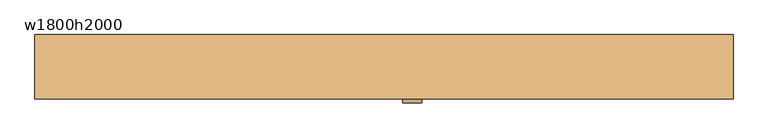
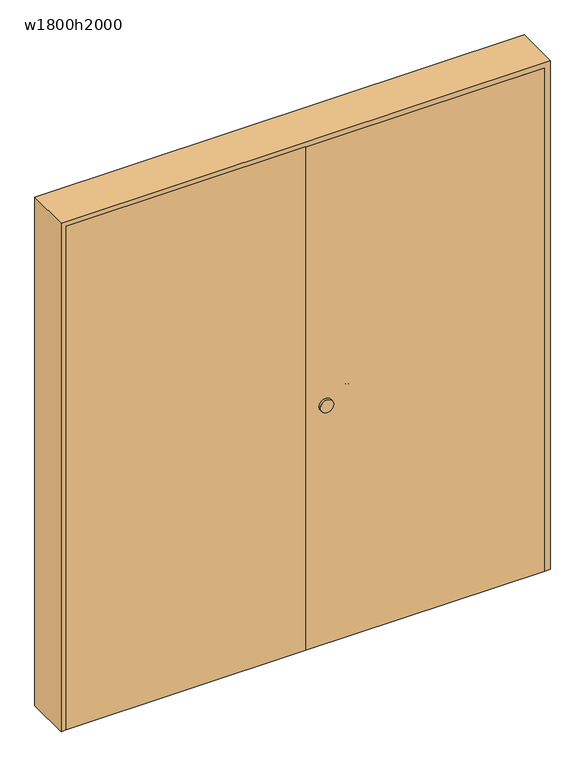
"""IFC4 building model written with IfcOpenShell, lengths in millimetres: door geometry, 二重 : w1800h2000."""

from ifc_helpers import new_model, si_unit, point, frame, frame_2d, origin, origin_with_axes, place, context, project, spatial, polyline, circle_curve, ellipse_curve, trimmed, segment, composite_curve, outline, extrude, source, transform, mapped, element, save
from ifc_brep_helpers import plane_surface, cylinder_surface, revolved_surface, advanced_brep


def w1800h2000_e7756d22(model_context):
    return source(origin(), model_context, "Body", "SolidModel", [
        advanced_brep(
        [(77.0, -45.0, 940.0), (82.0, -45.0, 945.0), (82.0, -45.0, 955.0), (77.0, -45.0, 960.0), (73.0, -45.0, 960.0), (68.0, -45.0, 955.0), (68.0, -45.0, 945.0), (73.0, -45.0, 940.0), (73.0, -10.0, 940.0), (85.0, 2.0, 940.0), (200.0, 2.0, 940.0), (212.0, -10.0, 940.0), (212.0, -15.0, 940.0), (208.0, -15.0, 940.0), (208.0, -10.0, 940.0), (200.0, -2.0, 940.0), (85.0, -2.0, 940.0), (77.0, -10.0, 940.0), (68.0, -10.0, 945.0), (68.0, -10.0, 955.0), (73.0, -10.0, 960.0), (77.0, -10.0, 960.0), (85.0, -2.0, 960.0), (200.0, -2.0, 960.0), (208.0, -10.0, 960.0), (208.0, -15.0, 960.0), (212.0, -15.0, 960.0), (212.0, -10.0, 960.0), (200.0, 2.0, 960.0), (85.0, 2.0, 960.0), (82.0, -10.0, 955.0), (82.0, -10.0, 945.0), (85.0, 7.0, 945.0), (85.0, 7.0, 955.0), (85.0, -7.0, 955.0), (85.0, -7.0, 945.0), (200.0, 7.0, 945.0), (200.0, 7.0, 955.0), (200.0, -7.0, 955.0), (200.0, -7.0, 945.0), (217.0, -10.0, 945.0), (217.0, -10.0, 955.0), (203.0, -10.0, 955.0), (203.0, -10.0, 945.0), (217.0, -15.0, 945.0), (217.0, -15.0, 955.0), (203.0, -15.0, 955.0), (203.0, -15.0, 945.0)],
        [
            (0, 1, circle_curve(frame((77.0, -45.0, 945.0), z_axis=(0.0, -1.0, 0.0), x_axis=(1.0, 0.0, 0.0)), 5.0)),
            (1, 2),
            (2, 3, circle_curve(frame((77.0, -45.0, 955.0), z_axis=(0.0, -1.0, 0.0), x_axis=(1.0, 0.0, 0.0)), 5.0)),
            (3, 4),
            (4, 5, circle_curve(frame((73.0, -45.0, 955.0), z_axis=(0.0, -1.0, 0.0), x_axis=(1.0, 0.0, 0.0)), 5.0)),
            (5, 6),
            (6, 7, circle_curve(frame((73.0, -45.0, 945.0), z_axis=(0.0, -1.0, 0.0), x_axis=(1.0, 0.0, 0.0)), 5.0)),
            (7, 0),
            (7, 8),
            (8, 9, circle_curve(frame((85.0, -10.0, 940.0), z_axis=(0.0, 0.0, -1.0), x_axis=(-1.0, 0.0, 0.0)), 12.0)),
            (9, 10),
            (10, 11, circle_curve(frame((200.0, -10.0, 940.0), z_axis=(0.0, 0.0, -1.0), x_axis=(0.0, 1.0, 0.0)), 12.0)),
            (11, 12),
            (12, 13),
            (13, 14),
            (14, 15, circle_curve(frame((200.0, -10.0, 940.0), z_axis=(0.0, 0.0, 1.0), x_axis=(0.0, 1.0, 0.0)), 8.0)),
            (15, 16),
            (16, 17, circle_curve(frame((85.0, -10.0, 940.0), z_axis=(0.0, 0.0, 1.0), x_axis=(-1.0, 0.0, 0.0)), 8.0)),
            (17, 0),
            (6, 18),
            (18, 8, circle_curve(frame((73.0, -10.0, 945.0), z_axis=(0.0, -1.0, 0.0), x_axis=(1.0, 0.0, 0.0)), 5.0)),
            (5, 19),
            (19, 18),
            (4, 20),
            (20, 19, circle_curve(frame((73.0, -10.0, 955.0), z_axis=(0.0, -1.0, 0.0), x_axis=(1.0, 0.0, 0.0)), 5.0)),
            (3, 21),
            (21, 22, circle_curve(frame((85.0, -10.0, 960.0), z_axis=(0.0, 0.0, -1.0), x_axis=(-1.0, 0.0, 0.0)), 8.0)),
            (22, 23),
            (23, 24, circle_curve(frame((200.0, -10.0, 960.0), z_axis=(0.0, 0.0, -1.0), x_axis=(0.0, 1.0, 0.0)), 8.0)),
            (24, 25),
            (25, 26),
            (26, 27),
            (27, 28, circle_curve(frame((200.0, -10.0, 960.0), z_axis=(0.0, 0.0, 1.0), x_axis=(0.0, 1.0, 0.0)), 12.0)),
            (28, 29),
            (29, 20, circle_curve(frame((85.0, -10.0, 960.0), z_axis=(0.0, 0.0, 1.0), x_axis=(-1.0, 0.0, 0.0)), 12.0)),
            (2, 30),
            (30, 21, circle_curve(frame((77.0, -10.0, 955.0), z_axis=(0.0, -1.0, 0.0), x_axis=(1.0, 0.0, 0.0)), 5.0)),
            (1, 31),
            (31, 30),
            (17, 31, circle_curve(frame((77.0, -10.0, 945.0), z_axis=(0.0, -1.0, 0.0), x_axis=(1.0, 0.0, 0.0)), 5.0)),
            (32, 9, circle_curve(frame((85.0, 2.0, 945.0), z_axis=(-1.0, 0.0, 0.0), x_axis=(0.0, -1.0, 0.0)), 5.0)),
            (18, 32, circle_curve(frame((85.0, -10.0, 945.0), z_axis=(0.0, 0.0, -1.0), x_axis=(-1.0, 0.0, 0.0)), 17.0)),
            (33, 32),
            (19, 33, circle_curve(frame((85.0, -10.0, 955.0), z_axis=(0.0, 0.0, -1.0), x_axis=(-1.0, 0.0, 0.0)), 17.0)),
            (29, 33, circle_curve(frame((85.0, 2.0, 955.0), z_axis=(-1.0, 0.0, 0.0), x_axis=(0.0, -1.0, 0.0)), 5.0)),
            (34, 22, circle_curve(frame((85.0, -2.0, 955.0), z_axis=(-1.0, 0.0, 0.0), x_axis=(0.0, -1.0, 0.0)), 5.0)),
            (30, 34, circle_curve(frame((85.0, -10.0, 955.0), z_axis=(0.0, 0.0, -1.0), x_axis=(-1.0, 0.0, 0.0)), 3.0)),
            (35, 34),
            (31, 35, circle_curve(frame((85.0, -10.0, 945.0), z_axis=(0.0, 0.0, -1.0), x_axis=(-1.0, 0.0, 0.0)), 3.0)),
            (16, 35, circle_curve(frame((85.0, -2.0, 945.0), z_axis=(-1.0, 0.0, 0.0), x_axis=(0.0, -1.0, 0.0)), 5.0)),
            (32, 36),
            (36, 10, circle_curve(frame((200.0, 2.0, 945.0), z_axis=(-1.0, 0.0, 0.0), x_axis=(0.0, -1.0, 0.0)), 5.0)),
            (33, 37),
            (37, 36),
            (28, 37, circle_curve(frame((200.0, 2.0, 955.0), z_axis=(-1.0, 0.0, 0.0), x_axis=(0.0, -1.0, 0.0)), 5.0)),
            (34, 38),
            (38, 23, circle_curve(frame((200.0, -2.0, 955.0), z_axis=(-1.0, 0.0, 0.0), x_axis=(0.0, -1.0, 0.0)), 5.0)),
            (35, 39),
            (39, 38),
            (15, 39, circle_curve(frame((200.0, -2.0, 945.0), z_axis=(-1.0, 0.0, 0.0), x_axis=(0.0, -1.0, 0.0)), 5.0)),
            (40, 11, circle_curve(frame((212.0, -10.0, 945.0), z_axis=(0.0, 1.0, 0.0), x_axis=(-1.0, 0.0, 0.0)), 5.0)),
            (36, 40, circle_curve(frame((200.0, -10.0, 945.0), z_axis=(0.0, 0.0, -1.0), x_axis=(0.0, 1.0, 0.0)), 17.0)),
            (41, 40),
            (37, 41, circle_curve(frame((200.0, -10.0, 955.0), z_axis=(0.0, 0.0, -1.0), x_axis=(0.0, 1.0, 0.0)), 17.0)),
            (27, 41, circle_curve(frame((212.0, -10.0, 955.0), z_axis=(0.0, 1.0, 0.0), x_axis=(-1.0, 0.0, 0.0)), 5.0)),
            (42, 24, circle_curve(frame((208.0, -10.0, 955.0), z_axis=(0.0, 1.0, 0.0), x_axis=(-1.0, 0.0, 0.0)), 5.0)),
            (38, 42, circle_curve(frame((200.0, -10.0, 955.0), z_axis=(0.0, 0.0, -1.0), x_axis=(0.0, 1.0, 0.0)), 3.0)),
            (43, 42),
            (39, 43, circle_curve(frame((200.0, -10.0, 945.0), z_axis=(0.0, 0.0, -1.0), x_axis=(0.0, 1.0, 0.0)), 3.0)),
            (14, 43, circle_curve(frame((208.0, -10.0, 945.0), z_axis=(0.0, 1.0, 0.0), x_axis=(-1.0, 0.0, 0.0)), 5.0)),
            (12, 44, circle_curve(frame((212.0, -15.0, 945.0), z_axis=(0.0, -1.0, 0.0), x_axis=(-1.0, 0.0, 0.0)), 5.0)),
            (44, 45),
            (45, 26, circle_curve(frame((212.0, -15.0, 955.0), z_axis=(0.0, -1.0, 0.0), x_axis=(-1.0, 0.0, 0.0)), 5.0)),
            (25, 46, circle_curve(frame((208.0, -15.0, 955.0), z_axis=(0.0, -1.0, 0.0), x_axis=(-1.0, 0.0, 0.0)), 5.0)),
            (46, 47),
            (47, 13, circle_curve(frame((208.0, -15.0, 945.0), z_axis=(0.0, -1.0, 0.0), x_axis=(-1.0, 0.0, 0.0)), 5.0)),
            (40, 44),
            (41, 45),
            (42, 46),
            (43, 47),
        ],
        [
            plane_surface(frame((64.801961, -45.0, 950.0), z_axis=(0.0, -1.0, 0.0), x_axis=(0.0, 0.0, -1.0))),
            plane_surface(frame((77.0, -45.0, 940.0), z_axis=(0.0, 0.0, -1.0), x_axis=(0.0, 1.0, 0.0))),
            cylinder_surface(frame((73.0, -45.0, 945.0), z_axis=(0.0, -1.0, 0.0), x_axis=(1.0, 0.0, 0.0)), 5.0),
            plane_surface(frame((68.0, -45.0, 945.0), z_axis=(-1.0, 0.0, 0.0), x_axis=(0.0, 1.0, 0.0))),
            cylinder_surface(frame((73.0, -45.0, 955.0), z_axis=(0.0, -1.0, 0.0), x_axis=(1.0, 0.0, 0.0)), 5.0),
            plane_surface(frame((73.0, -45.0, 960.0), z_axis=(0.0, 0.0, 1.0), x_axis=(0.0, 1.0, 0.0))),
            cylinder_surface(frame((77.0, -45.0, 955.0), z_axis=(0.0, -1.0, 0.0), x_axis=(1.0, 0.0, 0.0)), 5.0),
            plane_surface(frame((82.0, -45.0, 955.0), z_axis=(1.0, 0.0, 0.0), x_axis=(0.0, 1.0, 0.0))),
            cylinder_surface(frame((77.0, -45.0, 945.0), z_axis=(0.0, -1.0, 0.0), x_axis=(1.0, 0.0, 0.0)), 5.0),
            revolved_surface(trimmed(ellipse_curve(frame((73.0, -10.0, 945.0), z_axis=(0.0, 1.0, 0.0), x_axis=(1.0, 0.0, 0.0)), 5.0, 5.0), [point((73.0, -10.0, 940.0))], [point((68.0, -10.0, 945.0))], True, "CARTESIAN"), (85.0, -10.0, 950.0), (0.0, 0.0, 1.0)),
            cylinder_surface(frame((85.0, -10.0, 950.0), z_axis=(0.0, 0.0, 1.0), x_axis=(-1.0, 0.0, 0.0)), 17.0),
            revolved_surface(trimmed(ellipse_curve(frame((73.0, -10.0, 955.0), z_axis=(0.0, 1.0, 0.0), x_axis=(1.0, 0.0, 0.0)), 5.0, 5.0), [point((68.0, -10.0, 955.0))], [point((73.0, -10.0, 960.0))], True, "CARTESIAN"), (85.0, -10.0, 950.0), (0.0, 0.0, 1.0)),
            revolved_surface(trimmed(ellipse_curve(frame((77.0, -10.0, 955.0), z_axis=(0.0, 1.0, 0.0), x_axis=(1.0, 0.0, 0.0)), 5.0, 5.0), [point((77.0, -10.0, 960.0))], [point((82.0, -10.0, 955.0))], True, "CARTESIAN"), (85.0, -10.0, 950.0), (0.0, 0.0, 1.0)),
            revolved_surface(polyline([(82.0, -10.0, 955.0), (82.0, -10.0, 945.0)]), (85.0, -10.0, 950.0), (0.0, 0.0, 1.0)),
            revolved_surface(trimmed(ellipse_curve(frame((77.0, -10.0, 945.0), z_axis=(0.0, 1.0, 0.0), x_axis=(1.0, 0.0, 0.0)), 5.0, 5.0), [point((82.0, -10.0, 945.0))], [point((77.0, -10.0, 940.0))], True, "CARTESIAN"), (85.0, -10.0, 950.0), (0.0, 0.0, 1.0)),
            cylinder_surface(frame((85.0, 2.0, 945.0), z_axis=(-1.0, 0.0, 0.0), x_axis=(0.0, -1.0, 0.0)), 5.0),
            plane_surface(frame((85.0, 7.0, 945.0), z_axis=(0.0, 1.0, 0.0), x_axis=(1.0, 0.0, 0.0))),
            cylinder_surface(frame((85.0, 2.0, 955.0), z_axis=(-1.0, 0.0, 0.0), x_axis=(0.0, -1.0, 0.0)), 5.0),
            cylinder_surface(frame((85.0, -2.0, 955.0), z_axis=(-1.0, 0.0, 0.0), x_axis=(0.0, -1.0, 0.0)), 5.0),
            plane_surface(frame((85.0, -7.0, 955.0), z_axis=(0.0, -1.0, 0.0), x_axis=(1.0, 0.0, 0.0))),
            cylinder_surface(frame((85.0, -2.0, 945.0), z_axis=(-1.0, 0.0, 0.0), x_axis=(0.0, -1.0, 0.0)), 5.0),
            revolved_surface(trimmed(ellipse_curve(frame((200.0, 2.0, 945.0), z_axis=(1.0, 0.0, 0.0), x_axis=(0.0, -1.0, 0.0)), 5.0, 5.0), [point((200.0, 2.0, 940.0))], [point((200.0, 7.0, 945.0))], True, "CARTESIAN"), (200.0, -10.0, 950.0), (0.0, 0.0, 1.0)),
            cylinder_surface(frame((200.0, -10.0, 950.0), z_axis=(0.0, 0.0, 1.0), x_axis=(0.0, 1.0, 0.0)), 17.0),
            revolved_surface(trimmed(ellipse_curve(frame((200.0, 2.0, 955.0), z_axis=(1.0, 0.0, 0.0), x_axis=(0.0, -1.0, 0.0)), 5.0, 5.0), [point((200.0, 7.0, 955.0))], [point((200.0, 2.0, 960.0))], True, "CARTESIAN"), (200.0, -10.0, 950.0), (0.0, 0.0, 1.0)),
            revolved_surface(trimmed(ellipse_curve(frame((200.0, -2.0, 955.0), z_axis=(1.0, 0.0, 0.0), x_axis=(0.0, -1.0, 0.0)), 5.0, 5.0), [point((200.0, -2.0, 960.0))], [point((200.0, -7.0, 955.0))], True, "CARTESIAN"), (200.0, -10.0, 950.0), (0.0, 0.0, 1.0)),
            revolved_surface(polyline([(200.0, -7.0, 955.0), (200.0, -7.0, 945.0)]), (200.0, -10.0, 950.0), (0.0, 0.0, 1.0)),
            revolved_surface(trimmed(ellipse_curve(frame((200.0, -2.0, 945.0), z_axis=(1.0, 0.0, 0.0), x_axis=(0.0, -1.0, 0.0)), 5.0, 5.0), [point((200.0, -7.0, 945.0))], [point((200.0, -2.0, 940.0))], True, "CARTESIAN"), (200.0, -10.0, 950.0), (0.0, 0.0, 1.0)),
            plane_surface(frame((199.801961, -15.0, 950.0), z_axis=(0.0, -1.0, 0.0), x_axis=(0.0, 0.0, 1.0))),
            cylinder_surface(frame((212.0, -10.0, 945.0), z_axis=(0.0, 1.0, 0.0), x_axis=(-1.0, 0.0, 0.0)), 5.0),
            plane_surface(frame((217.0, -10.0, 945.0), z_axis=(1.0, 0.0, 0.0), x_axis=(0.0, -1.0, 0.0))),
            cylinder_surface(frame((212.0, -10.0, 955.0), z_axis=(0.0, 1.0, 0.0), x_axis=(-1.0, 0.0, 0.0)), 5.0),
            cylinder_surface(frame((208.0, -10.0, 955.0), z_axis=(0.0, 1.0, 0.0), x_axis=(-1.0, 0.0, 0.0)), 5.0),
            plane_surface(frame((203.0, -10.0, 955.0), z_axis=(-1.0, 0.0, 0.0), x_axis=(0.0, -1.0, 0.0))),
            cylinder_surface(frame((208.0, -10.0, 945.0), z_axis=(0.0, 1.0, 0.0), x_axis=(-1.0, 0.0, 0.0)), 5.0),
        ],
        [
            (0, [[1, 2, 3, 4, 5, 6, 7, 8]]),
            (1, [[9, 10, 11, 12, 13, 14, 15, 16, 17, 18, 19, -8]]),
            (2, [[20, 21, -9, -7]]),
            (3, [[22, 23, -20, -6]]),
            (4, [[24, 25, -22, -5]]),
            (5, [[26, 27, 28, 29, 30, 31, 32, 33, 34, 35, -24, -4]]),
            (6, [[36, 37, -26, -3]]),
            (7, [[38, 39, -36, -2]]),
            (8, [[-19, 40, -38, -1]]),
            (9, [[41, -10, -21, 42]]),
            (10, [[43, -42, -23, 44]]),
            (11, [[45, -44, -25, -35]]),
            (12, [[46, -27, -37, 47]]),
            (13, [[48, -47, -39, 49]]),
            (14, [[50, -49, -40, -18]]),
            (15, [[51, 52, -11, -41]]),
            (16, [[53, 54, -51, -43]]),
            (17, [[-34, 55, -53, -45]]),
            (18, [[56, 57, -28, -46]]),
            (19, [[58, 59, -56, -48]]),
            (20, [[-17, 60, -58, -50]]),
            (21, [[61, -12, -52, 62]]),
            (22, [[63, -62, -54, 64]]),
            (23, [[65, -64, -55, -33]]),
            (24, [[66, -29, -57, 67]]),
            (25, [[68, -67, -59, 69]]),
            (26, [[70, -69, -60, -16]]),
            (27, [[-14, 71, 72, 73, -31, 74, 75, 76]]),
            (28, [[77, -71, -13, -61]]),
            (29, [[78, -72, -77, -63]]),
            (30, [[-32, -73, -78, -65]]),
            (31, [[79, -74, -30, -66]]),
            (32, [[80, -75, -79, -68]]),
            (33, [[-15, -76, -80, -70]]),
        ],
    ),
        extrude(outline(composite_curve([segment(trimmed(circle_curve(frame_2d((950.0, 75.0)), 25.0), [point((950.0, 50.0))], [point((950.0, 100.0))], False, "CARTESIAN"), True, "CONTINUOUS"), segment(trimmed(circle_curve(frame_2d((950.0, 75.0)), 25.0), [point((950.0, 100.0))], [point((950.0, 50.0))], False, "CARTESIAN"), True, "CONTINUOUS")], self_intersect=False)), frame((0.0, -95.0, 0.0), z_axis=(0.0, 1.0, 0.0), x_axis=(0.0, 0.0, 1.0)), (0.0, 0.0, 1.0), 10.0),
        extrude(outline(composite_curve([segment(trimmed(circle_curve(frame_2d((950.0, 75.0)), 25.0), [point((950.0, 50.0))], [point((950.0, 100.0))], False, "CARTESIAN"), True, "CONTINUOUS"), segment(trimmed(circle_curve(frame_2d((950.0, 75.0)), 25.0), [point((950.0, 100.0))], [point((950.0, 50.0))], False, "CARTESIAN"), True, "CONTINUOUS")], self_intersect=False)), frame((0.0, -55.0, 0.0), z_axis=(0.0, 1.0, 0.0), x_axis=(0.0, 0.0, 1.0)), (0.0, 0.0, 1.0), 10.0),
        extrude(outline(polyline([(0.0, -55.0), (0.0, -85.0), (-900.0, -85.0), (-900.0, -55.0), (0.0, -55.0)])), origin_with_axes(), (0.0, 0.0, 1.0), 2000.0),
        extrude(outline(polyline([(2020.0, -920.0), (0.0, -920.0), (0.0, -900.0), (2000.0, -900.0), (2000.0, 900.0), (0.0, 900.0), (0.0, 920.0), (2020.0, 920.0), (2020.0, -920.0)])), frame((0.0, -85.0, 0.0), z_axis=(0.0, 1.0, 0.0), x_axis=(0.0, 0.0, 1.0)), (0.0, 0.0, 1.0), 170.0),
        extrude(outline(polyline([(900.0, -55.0), (900.0, -85.0), (0.0, -85.0), (0.0, -55.0), (900.0, -55.0)])), origin_with_axes(), (0.0, 0.0, 1.0), 2000.0),
    ])


if __name__ == "__main__":
    model = new_model("IFC4")
    model_context = context("Model", 3, world=origin())
    ifc_project = project(units=[si_unit("LENGTHUNIT", "METRE", prefix="MILLI")], contexts=[model_context])
    site = spatial("IfcSite", under=ifc_project)
    building = spatial("IfcBuilding", under=site)
    placement = place(None, origin())
    w1800h2000_shape = w1800h2000_e7756d22(model_context)
    element("IfcDoor", 1, ObjectType="二重 : w1800h2000", at=placement, inside=building, context=model_context, shape_type="MappedRepresentation", body=[
        mapped(w1800h2000_shape, transform((0.0, 0.0, 0.0), x_axis=(1.0, 0.0, 0.0), y_axis=(0.0, 1.0, 0.0), z_axis=(0.0, 0.0, 1.0))),
    ])
    save(model, "model.ifc")

# Revit data of these elements
# Project information
#   プロジェクト発行日 = "発行日"
#   プロジェクト ステータス = "プロジェクト ステータス"
#   クライアント名 = "オーナ"
#   計画地住所 = "ここにアドレスを入力"
#   プロジェクト名 = "プロジェクト名"
#   プロジェクト番号 = "0001"
# Type "二重 : w1800h2000"
#   Construction Type Id = "MDOOR"
#   Analytic Construction = "メタル"
#   Type Mark = "45"
#   Operation = "両開きドア単一スイング"
#   Keynote = "08110.R1"
#   Visual Light Transmittance = 0
#   Solar Heat Gain Coefficient = 0
#   Heat Transfer Coefficient (U) = 3.7021 W/(m²·K)
#   高さ(中心) = 1000 mm
#   Height = 2000 mm
#   Thickness = 30 mm
#   ドア枠見附 = 20 mm
#   Width = 1800 mm
#   取手取付け高さ = 950 mm
#   ドア枠ちり = 10 mm
#   Function = 0
#   ドア枠 [instance default] = none
#   ドア把手 [instance default] = メタル-ステンレス
#   ドア [instance default] = none
#   Wall Closure = (empty or 0)
# Element 1 (IfcDoor, "二重 : w1800h2000")
#   Materials on its faces: "メタル-ステンレス"
# Materials
#   "メタル-ステンレス": class "メタル", colour RGB 247 247 247, transparency 0, Cost = 0
